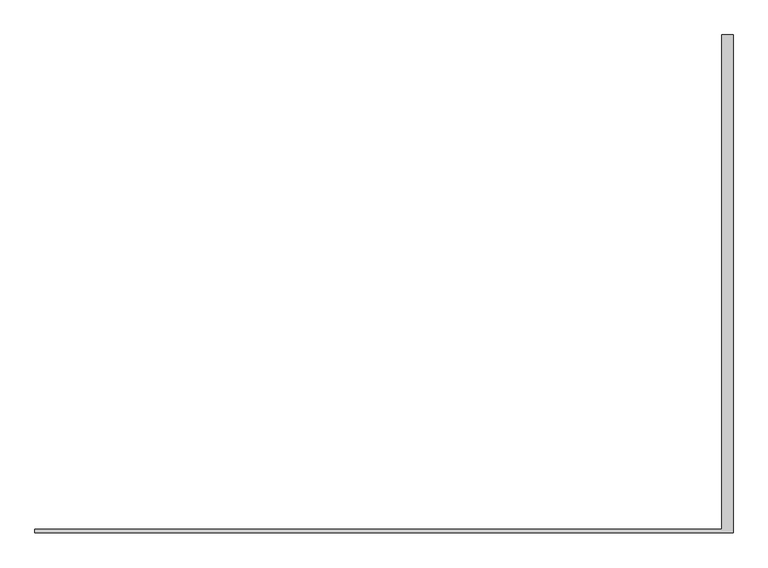
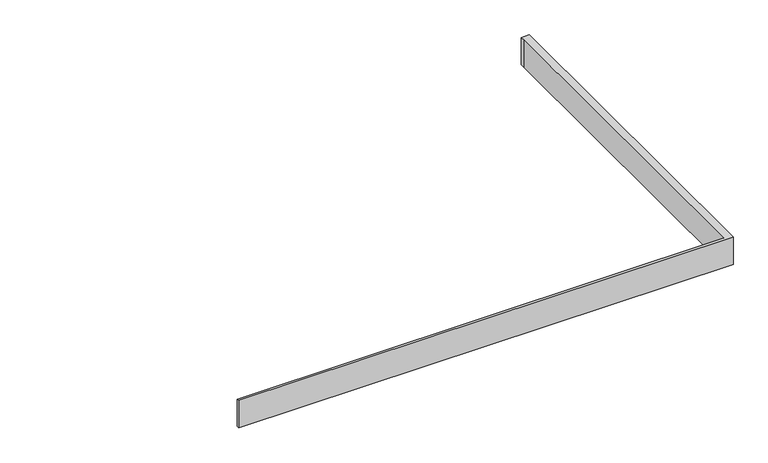
"""IFC4 building model written with IfcOpenShell, lengths in millimetres: furniture geometry, Kitchen - Main blacksplash : Kitchen - Main blacksplash."""

from ifc_helpers import new_model, si_unit, frame, origin, place, context, project, spatial, polyline, outline, extrude, source, transform, mapped, element, save


def furniture_3ef02292(model_context):
    return source(origin(), model_context, "Body", "SweptSolid", [
        extrude(outline(polyline([(5740.4, 8685.2125), (8302.625, 8685.2125), (8302.625, 10504.4875), (8302.625, 10529.8875), (8345.4875, 10529.8875), (8345.4875, 10504.4875), (8345.4875, 8672.5125), (5740.4, 8672.5125), (5740.4, 8685.2125)])), frame((0.0, 0.0, 914.3405752), z_axis=(0.0, 0.0, 1.0), x_axis=(1.0, 0.0, 0.0)), (0.0, 0.0, 1.0), 152.4594248),
    ])


if __name__ == "__main__":
    model = new_model("IFC4")
    model_context = context("Model", 3, world=origin())
    ifc_project = project(units=[si_unit("LENGTHUNIT", "METRE", prefix="MILLI")], contexts=[model_context])
    site = spatial("IfcSite", under=ifc_project)
    building = spatial("IfcBuilding", under=site)
    placement = place(None, origin())
    furniture_shape = furniture_3ef02292(model_context)
    element("IfcFurniture", 1, ObjectType="Kitchen - Main blacksplash : Kitchen - Main blacksplash", at=placement, inside=building, context=model_context, shape_type="MappedRepresentation", body=[
        mapped(furniture_shape, transform((0.0, 0.0, 0.0), x_axis=(1.0, 0.0, 0.0), y_axis=(0.0, 1.0, 0.0), z_axis=(0.0, 0.0, 1.0))),
    ])
    save(model, "model.ifc")

# Revit data of these elements
# Type "Kitchen - Main blacksplash : Kitchen - Main blacksplash"
#   COBie.Type = no
# Element 1 (IfcFurniture, "Kitchen - Main blacksplash : Kitchen - Main blacksplash")
#   Materials on its faces: "Corian - Dusk"
# Materials
#   "Corian - Dusk": class "Plastic", colour RGB 75 95 146, transparency 0, Manufacturer = "Corning", Cost = 0
